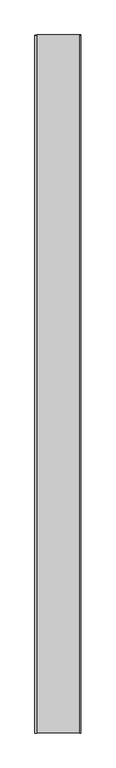
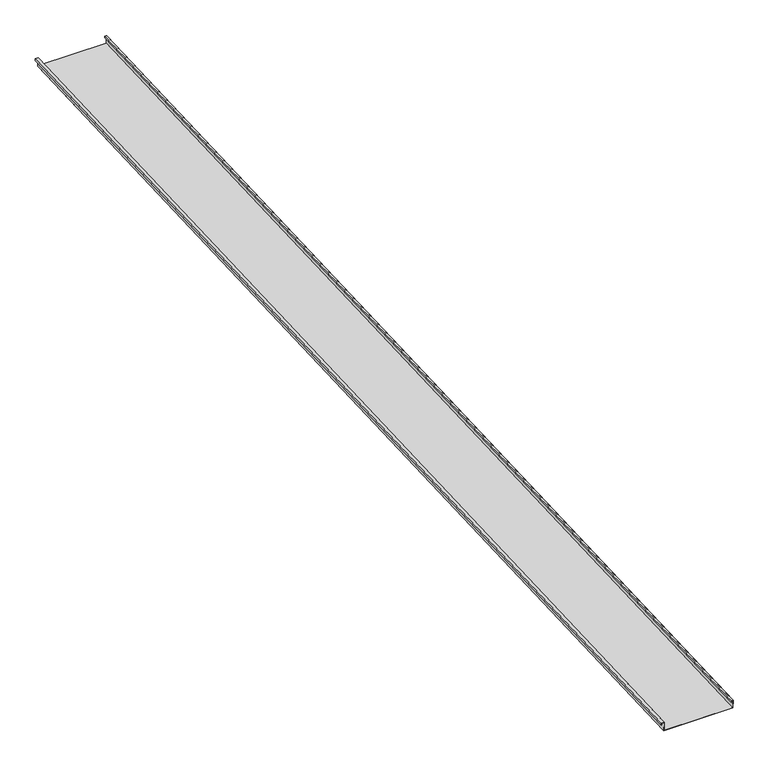
"""IFC4 building model written with IfcOpenShell, lengths in millimetres: proxy geometry, Generic Models 2:Generic Models 2:310765:Generic Models 2:310765 : Generic Models 2:Generic Models 2:310765:95 : Generic Models 2:Generic Models 2:310765:Generic Models 2:310765 : Generic Models 2:Generic Models 2:310765:300385."""

from ifc_helpers import new_model, si_unit, frame, origin, place, context, project, spatial, polyline, outline, extrude, source, transform, mapped, element, save


def generic_models_e730b164(model_context):
    return source(origin(), model_context, "Body", "SweptSolid", [
        extrude(outline(polyline([(1.5875, 0.0), (1.5875, 50.8), (407.9875, 50.8), (407.9875, 1.5875), (396.875, 1.5875), (396.875, 11.1125), (398.4625, 11.1125), (398.4625, 3.175), (406.4, 3.175), (406.4, 49.2125), (3.175, 49.2125), (3.175, -1.5874999), (-14.2875, -1.5874999), (-14.2875, 9.525), (-12.7, 9.525), (-12.7, 0.0), (1.5875, 0.0)])), frame((615187.5929739, -581354.4345603, 3902.6697972), z_axis=(0.0, 0.9991330730923568, 0.041630544712067834), x_axis=(1.0, 0.0, 0.0)), (0.0, 0.0, 1.0), 6400.8),
    ])


if __name__ == "__main__":
    model = new_model("IFC4")
    model_context = context("Model", 3, world=origin())
    ifc_project = project(units=[si_unit("LENGTHUNIT", "METRE", prefix="MILLI")], contexts=[model_context])
    site = spatial("IfcSite", under=ifc_project)
    building = spatial("IfcBuilding", under=site)
    placement = place(None, origin())
    generic_models_shape = generic_models_e730b164(model_context)
    element("IfcBuildingElementProxy", 1, Name="Generic Models 2:Generic Models 2:310765:Generic Models 2:310765 : Generic Models 2:Generic Models 2:310765:95 : Generic Models 2:Generic Models 2:310765:Generic Models 2:310765 : Generic Models 2:Generic Models 2:310765:300385", ObjectType="Generic Models 2:Generic Models 2:310765:Generic Models 2:310765 : Generic Models 2:Generic Models 2:310765:95 : Generic Models 2:Generic Models 2:310765:Generic Models 2:310765 : Generic Models 2:Generic Models 2:310765:300385", at=placement, inside=building, context=model_context, shape_type="MappedRepresentation", body=[
        mapped(generic_models_shape, transform((0.0, 0.0, 0.0), x_axis=(1.0, 0.0, 0.0), y_axis=(0.0, 1.0, 0.0), z_axis=(0.0, 0.0, 1.0))),
    ])
    save(model, "model.ifc")

# Revit data of these elements
# Type "Generic Models 2:Generic Models 2:310765:Generic Models 2:310765 : Generic Models 2:Generic Models 2:310765:95 : Generic Models 2:Generic Models 2:310765:Generic Models 2:310765 : Generic Models 2:Generic Models 2:310765:300385"
#   NameOverride = "Generic Models 2:Generic Models 2:310765:Generic Models 2:310765 : Generic Models 2:Generic Models 2:310765:300385"
#   ObjectTypeOverride = "Generic Models 2:310765 : Generic Models 2:Generic Models 2:310765"
#   Reference = "Generic Models 2"
#   Tag = "300385"
# Element 1 (IfcBuildingElementProxy, "Generic Models 2:Generic Models 2:310765:Generic Models 2:310765 : Generic Models 2:Generic Models 2:310765:95 : Generic Models 2:Generic Models 2:310765:Generic Models 2:310765 : Generic Models 2:Generic Models 2:310765:300385")
#   Materials on its faces: "THERMAL BROKEN ALUMINUM STOREFRONT FOR POLYCARBONATE"
# Materials
#   "THERMAL BROKEN ALUMINUM STOREFRONT FOR POLYCARBONATE": class "Unassigned", colour RGB 244 244 244, transparency 0, Keynote = "M07611300.01", Cost = 0
